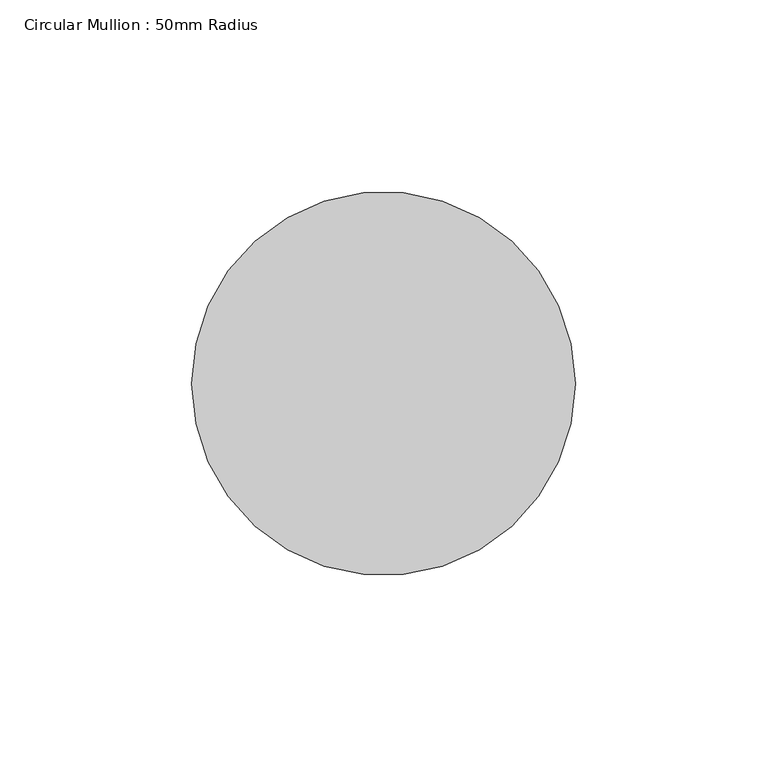
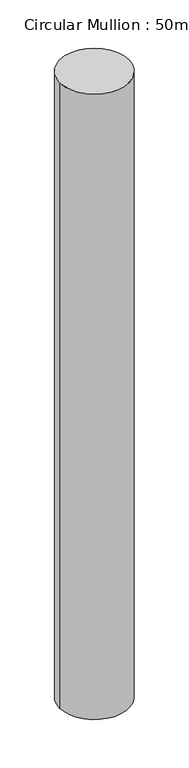
"""IFC4 building model written with IfcOpenShell, lengths in millimetres: member geometry, Circular Mullion : 50mm Radius."""

from ifc_helpers import new_model, si_unit, point, frame, origin, origin_2d, place, context, project, spatial, circle_curve, trimmed, segment, composite_curve, outline, extrude, source, transform, mapped, element, save


def circular_mullion_50mm_radius_904c3a7f(model_context):
    return source(origin(), model_context, "Body", "SweptSolid", [
        extrude(outline(composite_curve([segment(trimmed(circle_curve(origin_2d(), 50.0), [point((50.0, 0.0))], [point((-50.0, 0.0))], False, "CARTESIAN"), True, "CONTINUOUS"), segment(trimmed(circle_curve(origin_2d(), 50.0), [point((-50.0, 0.0))], [point((50.0, 0.0))], False, "CARTESIAN"), True, "CONTINUOUS")], self_intersect=False)), frame((0.0, 0.0, -955.0572644), z_axis=(0.0, 0.0, 1.0), x_axis=(1.0, 0.0, 0.0)), (0.0, 0.0, 1.0), 955.0572644),
    ])


if __name__ == "__main__":
    model = new_model("IFC4")
    model_context = context("Model", 3, world=origin())
    ifc_project = project(units=[si_unit("LENGTHUNIT", "METRE", prefix="MILLI")], contexts=[model_context])
    site = spatial("IfcSite", under=ifc_project)
    building = spatial("IfcBuilding", under=site)
    placement = place(None, origin())
    circular_mullion_50mm_radius_shape = circular_mullion_50mm_radius_904c3a7f(model_context)
    element("IfcMember", 1, ObjectType="Circular Mullion : 50mm Radius", at=placement, inside=building, context=model_context, shape_type="MappedRepresentation", body=[
        mapped(circular_mullion_50mm_radius_shape, transform((0.0, 0.0, 0.0), x_axis=(1.0, 0.0, 0.0), y_axis=(0.0, 1.0, 0.0), z_axis=(0.0, 0.0, 1.0))),
    ])
    save(model, "model.ifc")

# Revit data of these elements
# Type "Circular Mullion : 50mm Radius"
#   built-in parameter 1007350 = 0.164042 (stored number, unit not read)
# Element 1 (IfcMember, "Circular Mullion : 50mm Radius")
#   Materials on its faces: "Aluminium"
# Materials
#   "Aluminium": class "Metal", colour RGB 247 247 247, transparency 0, Description = "Aluminium 6061", Cost = 0
